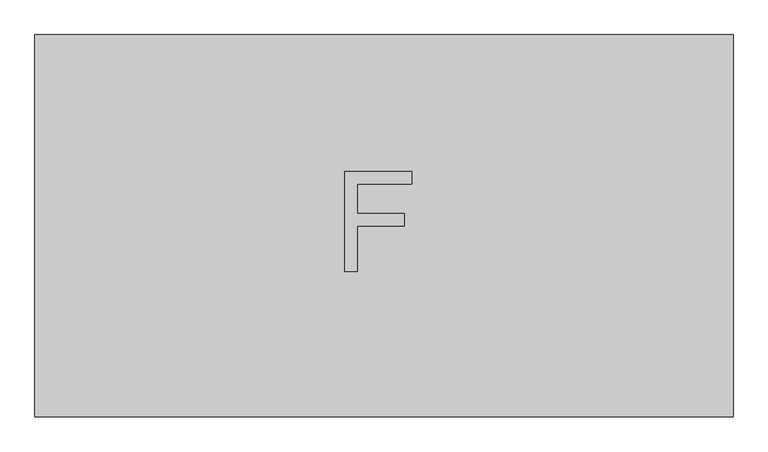
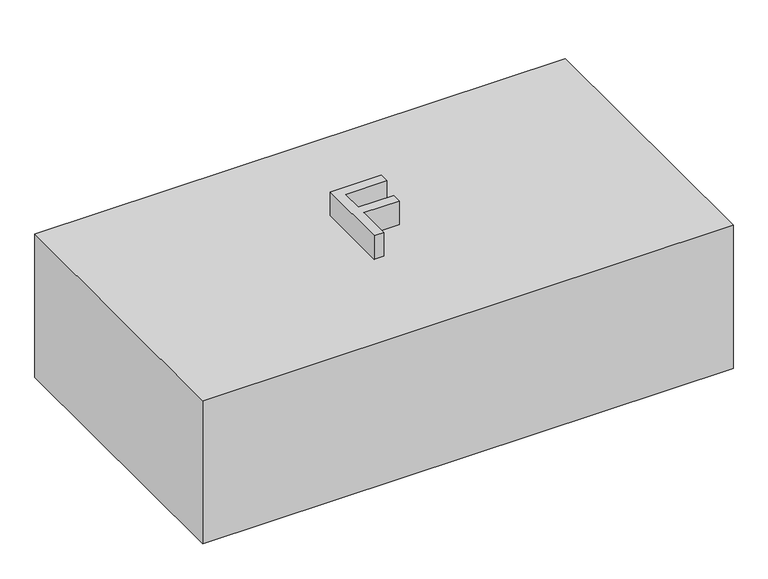
"""IFC4 building model written with IfcOpenShell, lengths in millimetres: proxy geometry, The Messy Family F : The Messy Family F."""

import ifcopenshell
import ifcopenshell.guid

model = None  # the IFC model being written
_history = None  # IfcOwnerHistory: only IFC2X3 demands one
_inside = {}  # id of a spatial element -> (the spatial element, [elements in it])
_under = {}  # id of a project, library or spatial element -> (it, [spatial elements below it])
_declared = {}  # id of a project -> (the project, [libraries it declares])
_typed = {}  # id of a type object -> (the type object, [elements of that type])
_made_of = {}  # id of a material, layer set ... -> (it, [elements and type objects made of it])


def new_model(schema):
    """Start an empty IFC model of exactly this schema.

    Asked for "IFC4X3", IfcOpenShell would pick the latest addendum, in which some entities
    have other attributes; the version numbers below select the first issue.
    IFC2X3 requires an IfcOwnerHistory on every rooted entity: one is made here for all.
    """
    global model, _history
    if schema == "IFC4X3":
        model = ifcopenshell.file(schema_version=(4, 3, 0, 0))
    else:
        model = ifcopenshell.file(schema=schema)
    _inside.clear()
    _under.clear()
    _declared.clear()
    _typed.clear()
    _made_of.clear()
    _history = None
    if model.schema == "IFC2X3":
        org = make("IfcOrganization", Name="unknown")
        user = make(
            "IfcPersonAndOrganization",
            ThePerson=make("IfcPerson", FamilyName="unknown"),
            TheOrganization=org,
        )
        app = make(
            "IfcApplication",
            ApplicationDeveloper=org,
            Version="unknown",
            ApplicationFullName="unknown",
            ApplicationIdentifier="unknown",
        )
        _history = make(
            "IfcOwnerHistory",
            OwningUser=user,
            OwningApplication=app,
            ChangeAction="ADDED",
            CreationDate=0,
        )
    return model


def make(cls, **values):
    """One entity of the class cls with the attributes given. An attribute that is None is left unset."""
    return model.create_entity(
        cls, **{name: value for name, value in values.items() if value is not None}
    )


def rooted(cls, **values):
    """An entity with a GlobalId (a new one), such as an element, a storey or a relation."""
    return make(cls, GlobalId=ifcopenshell.guid.new(), OwnerHistory=_history, **values)


def si_unit(unit_type, name, prefix=None):
    """IfcSIUnit, for example si_unit("LENGTHUNIT", "METRE", prefix="MILLI")."""
    return make("IfcSIUnit", UnitType=unit_type, Prefix=prefix, Name=name)


def assignment(units):
    """IfcUnitAssignment: the units of a project."""
    return None if units is None else make("IfcUnitAssignment", Units=units)


def point(xyz):
    """IfcCartesianPoint."""
    return None if xyz is None else make("IfcCartesianPoint", Coordinates=xyz)


def direction(xyz):
    """IfcDirection."""
    return None if xyz is None else make("IfcDirection", DirectionRatios=xyz)


def frame(location, z_axis=None, x_axis=None):
    """IfcAxis2Placement3D, a coordinate frame: its origin and axes. An axis left out is left unset."""
    return make(
        "IfcAxis2Placement3D",
        Location=point(location),
        Axis=direction(z_axis),
        RefDirection=direction(x_axis),
    )


def origin():
    """The frame at (0, 0, 0) with its axes left unset."""
    return frame((0.0, 0.0, 0.0))


def origin_with_axes():
    """The frame at (0, 0, 0) with the z axis (0, 0, 1) and the x axis (1, 0, 0) written out."""
    return frame((0.0, 0.0, 0.0), z_axis=(0.0, 0.0, 1.0), x_axis=(1.0, 0.0, 0.0))


def place(relative_to, where):
    """IfcLocalPlacement: puts the frame where relative to a parent placement (None: the world)."""
    return make(
        "IfcLocalPlacement", PlacementRelTo=relative_to, RelativePlacement=where
    )


def context(
    kind, dimensions, precision=None, world=None, true_north=None, identifier=None
):
    """IfcGeometricRepresentationContext, for example the 3D "Model" context."""
    return make(
        "IfcGeometricRepresentationContext",
        ContextIdentifier=identifier,
        ContextType=kind,
        CoordinateSpaceDimension=dimensions,
        Precision=precision,
        WorldCoordinateSystem=world,
        TrueNorth=true_north,
    )


def project(units=None, contexts=None):
    """IfcProject with its units and contexts."""
    return rooted(
        "IfcProject",
        Name="project",
        RepresentationContexts=contexts,
        UnitsInContext=assignment(units),
    )


def spatial(cls, under=None, at=None, **own):
    """A site, building, storey or space (cls), placed at a placement, below another one or the project."""
    s = rooted(cls, ObjectPlacement=at, **own)
    if under is not None:
        _under.setdefault(under.id(), (under, []))[1].append(s)
    return s


def polyline(points):
    """IfcPolyline through the points."""
    return make("IfcPolyline", Points=[point(p) for p in points])


def outline(outer, holes=None, kind="AREA"):
    """IfcArbitraryClosedProfileDef: a profile drawn as a closed curve; with holes, ...WithVoids."""
    if holes is None:
        return make("IfcArbitraryClosedProfileDef", ProfileType=kind, OuterCurve=outer)
    return make(
        "IfcArbitraryProfileDefWithVoids",
        ProfileType=kind,
        OuterCurve=outer,
        InnerCurves=holes,
    )


def extrude(swept, where, along, depth):
    """IfcExtrudedAreaSolid: the profile swept, set in the frame where, extruded along a direction by depth."""
    return make(
        "IfcExtrudedAreaSolid",
        SweptArea=swept,
        Position=where,
        ExtrudedDirection=direction(along),
        Depth=depth,
    )


def shape(context_of_items, identifier, shape_type, items):
    """IfcShapeRepresentation: the items that make up one representation, for example the "Body"."""
    return make(
        "IfcShapeRepresentation",
        ContextOfItems=context_of_items,
        RepresentationIdentifier=identifier,
        RepresentationType=shape_type,
        Items=items,
    )


def source(mapping_origin, context_of_items, identifier, shape_type, items):
    """IfcRepresentationMap: a shape defined once, which mapped items show again and again."""
    return make(
        "IfcRepresentationMap",
        MappingOrigin=mapping_origin,
        MappedRepresentation=shape(context_of_items, identifier, shape_type, items),
    )


def transform(
    local_origin,
    x_axis=None,
    y_axis=None,
    z_axis=None,
    scale=None,
    scale2=None,
    scale3=None,
    uniform=True,
):
    """IfcCartesianTransformationOperator3D, or its non-uniform kind. x_axis, y_axis, z_axis: its Axis1, 2, 3."""
    if uniform:
        return make(
            "IfcCartesianTransformationOperator3D",
            Axis1=direction(x_axis),
            Axis2=direction(y_axis),
            LocalOrigin=point(local_origin),
            Scale=scale,
            Axis3=direction(z_axis),
        )
    return make(
        "IfcCartesianTransformationOperator3DnonUniform",
        Axis1=direction(x_axis),
        Axis2=direction(y_axis),
        LocalOrigin=point(local_origin),
        Scale=scale,
        Axis3=direction(z_axis),
        Scale2=scale2,
        Scale3=scale3,
    )


def mapped(mapping_source, mapping_target):
    """IfcMappedItem: shows the shape of a source again, moved by a transform."""
    return make(
        "IfcMappedItem", MappingSource=mapping_source, MappingTarget=mapping_target
    )


def made_of(thing, what):
    """Note that an element or type object is made of a material, layer set ...; save() writes the relation."""
    if what is not None:
        _made_of.setdefault(what.id(), (what, []))[1].append(thing)
    return thing


def element(
    cls,
    number,
    at=None,
    inside=None,
    cuts=None,
    type_object=None,
    material=None,
    context=None,
    identifier="Body",
    shape_type=None,
    held_by="IfcProductDefinitionShape",
    body=None,
    shapes=None,
    **own,
):
    """One element of the class cls, such as IfcWall. Its Tag is "e" and its number.

    at: its placement. inside: the storey or other place that contains it. cuts: it is an
    opening in that element (IfcRelVoidsElement). A single representation is given by context,
    identifier, shape_type and body (its items); several are given by shapes. held_by: the class
    of the entity that holds the representations. save() writes the other relations.
    """
    e = rooted(cls, Tag="e%d" % number, ObjectPlacement=at, **own)
    if body is not None:
        shapes = [shape(context, identifier, shape_type, body)]
    if shapes is not None:
        e.Representation = make(held_by, Representations=shapes)
    if inside is not None:
        _inside.setdefault(inside.id(), (inside, []))[1].append(e)
    if cuts is not None:
        rooted(
            "IfcRelVoidsElement", RelatingBuildingElement=cuts, RelatedOpeningElement=e
        )
    if type_object is not None:
        _typed.setdefault(type_object.id(), (type_object, []))[1].append(e)
    return made_of(e, material)


def aggregate(whole, parts):
    """IfcRelAggregates: a whole, such as a stair, and the parts it consists of."""
    return rooted("IfcRelAggregates", RelatingObject=whole, RelatedObjects=parts)


def save(model, path):
    """Write the relations noted so far, then the file.

    IfcRelAggregates (storeys below a building ...), IfcRelContainedInSpatialStructure (elements
    in a storey), IfcRelDefinesByType, IfcRelAssociatesMaterial and IfcRelDeclares: one each for
    every whole, place, type object, material and project.
    """
    for whole, parts in _under.values():
        aggregate(whole, parts)
    for where, things in _inside.values():
        rooted(
            "IfcRelContainedInSpatialStructure",
            RelatedElements=things,
            RelatingStructure=where,
        )
    for kind, things in _typed.values():
        rooted("IfcRelDefinesByType", RelatedObjects=things, RelatingType=kind)
    for what, things in _made_of.values():
        rooted("IfcRelAssociatesMaterial", RelatedObjects=things, RelatingMaterial=what)
    for by, libraries in _declared.values():
        rooted("IfcRelDeclares", RelatingContext=by, RelatedDefinitions=libraries)
    model.write(path)


def generic_models_c7bdb3ab(model_context):
    return source(origin(), model_context, "Body", "SweptSolid", [
        extrude(outline(polyline([(541.9415527, 284.565081), (541.9415527, -299.634919), (-524.8584473, -299.634919), (-524.8584473, 284.565081), (541.9415527, 284.565081)])), origin_with_axes(), (0.0, 0.0, 1.0), 304.8),
        extrude(outline(polyline([(-51.7602961, -77.2556777), (-51.7602961, 75.839739), (51.100687, 75.839739), (51.100687, 56.7028119), (-32.623369, 56.7028119), (-32.623369, 11.2526101), (39.1401076, 11.2526101), (39.1401076, -7.884317), (-32.623369, -7.884317), (-32.623369, -77.2556777), (-51.7602961, -77.2556777)])), frame((0.0, 0.0, 304.8), z_axis=(0.0, 0.0, 1.0), x_axis=(1.0, 0.0, 0.0)), (0.0, 0.0, 1.0), 50.8),
    ])


if __name__ == "__main__":
    model = new_model("IFC4")
    model_context = context("Model", 3, world=origin())
    ifc_project = project(units=[si_unit("LENGTHUNIT", "METRE", prefix="MILLI")], contexts=[model_context])
    site = spatial("IfcSite", under=ifc_project)
    building = spatial("IfcBuilding", under=site)
    placement = place(None, origin())
    generic_models_shape = generic_models_c7bdb3ab(model_context)
    element("IfcBuildingElementProxy", 1, Name="The Messy Family F : The Messy Family F", ObjectType="The Messy Family F : The Messy Family F", at=placement, inside=building, context=model_context, shape_type="MappedRepresentation", body=[
        mapped(generic_models_shape, transform((0.0, 0.0, 0.0), x_axis=(1.0, 0.0, 0.0), y_axis=(0.0, 1.0, 0.0), z_axis=(0.0, 0.0, 1.0))),
    ])
    save(model, "model.ifc")

# Revit data of these elements
# Type "The Messy Family F : The Messy Family F"
#   TBC-Parameter 2 = ""
#   TBC-Parameter 1 = ""
#   Other Company Parameter 2 = ""
#   Other Company Parameter 1 = ""
#   TBC-Parameter 3 = 2' - 0"
#   Other Company Parameter 3 = 1' - 0"
#   Default Elevation = 0
